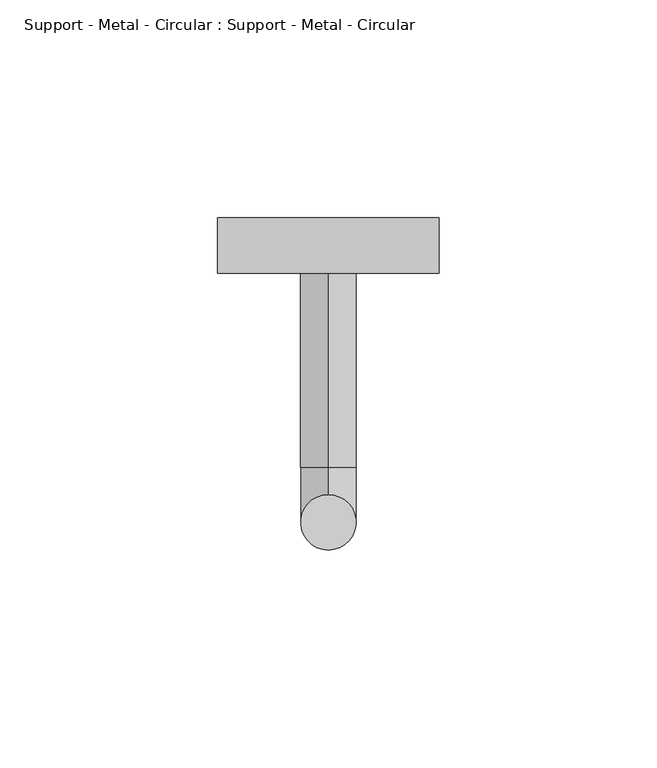
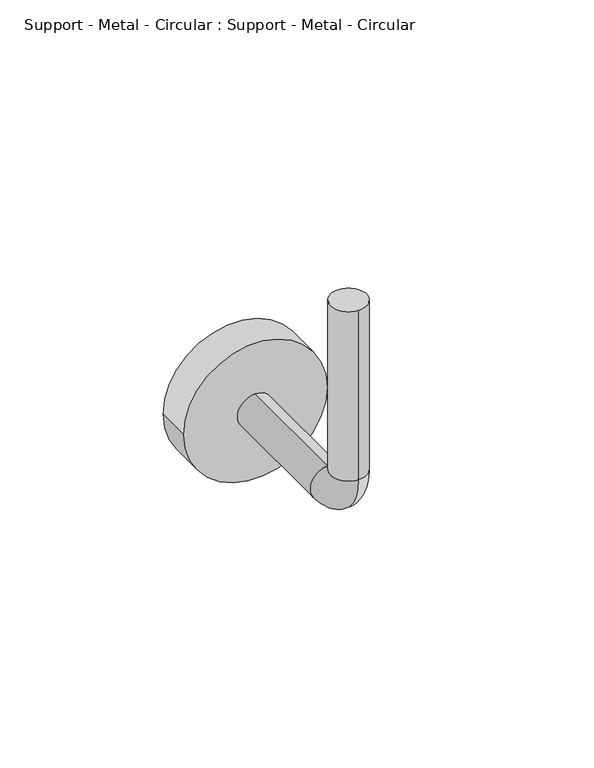
"""IFC4 building model written with IfcOpenShell, lengths in millimetres: proxy geometry, Support - Metal - Circular : Support - Metal - Circular."""

from ifc_helpers import new_model, si_unit, point, frame, frame_2d, origin, origin_with_axes, place, context, project, spatial, circle_curve, ellipse_curve, trimmed, segment, composite_curve, outline, extrude, source, transform, mapped, element, save
from ifc_brep_helpers import plane_surface, cylinder_surface, revolved_surface, advanced_brep


def support_metal_circular_support_metal_circular_b7c6dc0a(model_context):
    return source(origin(), model_context, "Body", "SolidModel", [
        advanced_brep(
        [(0.0, 57.15, -69.85), (0.0, 57.15, -82.55), (0.0, 12.7, -69.85), (0.0, 12.7, -82.55), (0.0, -6.35, -63.5), (0.0, 6.35, -63.5), (0.0, 6.35, 0.0), (0.0, -6.35, 0.0)],
        [
            (0, 1, circle_curve(frame((0.0, 57.15, -76.2), z_axis=(0.0, 1.0, 0.0), x_axis=(0.0, 0.0, -1.0)), 6.35)),
            (1, 0, circle_curve(frame((0.0, 57.15, -76.2), z_axis=(0.0, 1.0, 0.0), x_axis=(0.0, 0.0, -1.0)), 6.35)),
            (0, 2),
            (2, 3, circle_curve(frame((0.0, 12.7, -76.2), z_axis=(0.0, 1.0, 0.0), x_axis=(0.0, 0.0, -1.0)), 6.35)),
            (3, 1),
            (3, 2, circle_curve(frame((0.0, 12.7, -76.2), z_axis=(0.0, 1.0, 0.0), x_axis=(0.0, 0.0, -1.0)), 6.35)),
            (4, 3, circle_curve(frame((0.0, 12.7, -63.5), z_axis=(1.0, 0.0, 0.0), x_axis=(0.0, 0.0, -1.0)), 19.05)),
            (2, 5, circle_curve(frame((0.0, 12.7, -63.5), z_axis=(-1.0, 0.0, 0.0), x_axis=(0.0, 0.0, -1.0)), 6.35)),
            (5, 4, circle_curve(frame((0.0, 0.0, -63.5), z_axis=(0.0, 0.0, -1.0), x_axis=(0.0, -1.0, 0.0)), 6.35)),
            (4, 5, circle_curve(frame((0.0, 0.0, -63.5), z_axis=(0.0, 0.0, -1.0), x_axis=(0.0, -1.0, 0.0)), 6.35)),
            (6, 7, circle_curve(frame((0.0, 0.0, 0.0), z_axis=(0.0, 0.0, 1.0), x_axis=(0.0, -1.0, 0.0)), 6.35)),
            (7, 6, circle_curve(frame((0.0, 0.0, 0.0), z_axis=(0.0, 0.0, 1.0), x_axis=(0.0, -1.0, 0.0)), 6.35)),
            (5, 6),
            (7, 4),
        ],
        [
            plane_surface(frame((0.0, 57.15, -76.2), z_axis=(0.0, 1.0, 0.0), x_axis=(1.0, 0.0, 0.0))),
            cylinder_surface(frame((0.0, 57.15, -76.2), z_axis=(0.0, 1.0, 0.0), x_axis=(0.0, 0.0, -1.0)), 6.35),
            revolved_surface(trimmed(ellipse_curve(frame((0.0, 12.7, -76.2), z_axis=(0.0, 1.0, 0.0), x_axis=(0.0, 0.0, -1.0)), 6.35, 6.35), [point((0.0, 12.7, -69.85))], [point((0.0, 12.7, -82.55))], True, "CARTESIAN"), (0.0, 12.7, -63.5), (-1.0, 0.0, 0.0)),
            revolved_surface(trimmed(ellipse_curve(frame((0.0, 12.7, -76.2), z_axis=(0.0, 1.0, 0.0), x_axis=(0.0, 0.0, -1.0)), 6.35, 6.35), [point((0.0, 12.7, -82.55))], [point((0.0, 12.7, -69.85))], True, "CARTESIAN"), (0.0, 12.7, -63.5), (-1.0, 0.0, 0.0)),
            plane_surface(origin_with_axes()),
            cylinder_surface(frame((0.0, 0.0, -63.5), z_axis=(0.0, 0.0, -1.0), x_axis=(0.0, -1.0, 0.0)), 6.35),
        ],
        [
            (0, [[1, 2]]),
            (1, [[-1, 3, 4, 5]]),
            (1, [[-2, -5, 6, -3]]),
            (2, [[7, -4, 8, 9]]),
            (3, [[-8, -6, -7, 10]]),
            (4, [[11, 12]]),
            (5, [[-9, 13, -12, 14]]),
            (5, [[-10, -14, -11, -13]]),
        ],
    ),
        extrude(outline(composite_curve([segment(trimmed(circle_curve(frame_2d((-76.2, 0.0)), 25.4), [point((-76.2, -25.4))], [point((-76.2, 25.4))], False, "CARTESIAN"), True, "CONTINUOUS"), segment(trimmed(circle_curve(frame_2d((-76.2, 0.0)), 25.4), [point((-76.2, 25.4))], [point((-76.2, -25.4))], False, "CARTESIAN"), True, "CONTINUOUS")], self_intersect=False)), frame((0.0, 57.15, 0.0), z_axis=(0.0, 1.0, 0.0), x_axis=(0.0, 0.0, 1.0)), (0.0, 0.0, 1.0), 12.7),
    ])


if __name__ == "__main__":
    model = new_model("IFC4")
    model_context = context("Model", 3, world=origin())
    ifc_project = project(units=[si_unit("LENGTHUNIT", "METRE", prefix="MILLI")], contexts=[model_context])
    site = spatial("IfcSite", under=ifc_project)
    building = spatial("IfcBuilding", under=site)
    placement = place(None, origin())
    support_metal_circular_support_metal_circular_shape = support_metal_circular_support_metal_circular_b7c6dc0a(model_context)
    element("IfcBuildingElementProxy", 1, Name="Support - Metal - Circular : Support - Metal - Circular", ObjectType="Support - Metal - Circular : Support - Metal - Circular", at=placement, inside=building, context=model_context, shape_type="MappedRepresentation", body=[
        mapped(support_metal_circular_support_metal_circular_shape, transform((0.0, 0.0, 0.0), x_axis=(1.0, 0.0, 0.0), y_axis=(0.0, 1.0, 0.0), z_axis=(0.0, 0.0, 1.0))),
    ])
    save(model, "model.ifc")

# Revit data of these elements
# Type "Support - Metal - Circular : Support - Metal - Circular"
#   T1 = 0' - 0 1/2"
#   Radius 1 = 0' - 1"
#   Radius 2 = 0' - 0 1/4"
#   built-in parameter 1152166 = 0.25 (stored number, unit not read)
#   built-in parameter 1152165 [instance default] = 0.25 (stored number, unit not read)
#   Bend Radius = 0' - 0 1/2"
#   Support Material = KAWNEER TRIFAB VERSAGLAZE 451T - CLEAR ANODIZED ALUM. - BACK GLAZED
# Element 1 (IfcBuildingElementProxy, "Support - Metal - Circular : Support - Metal - Circular")
#   built-in parameter 1152165 = 0.229167 (stored number, unit not read)
#   Materials on its faces: "KAWNEER TRIFAB VERSAGLAZE 451T - CLEAR ANODIZED ALUM. - BACK GLAZED"
# Materials
#   "KAWNEER TRIFAB VERSAGLAZE 451T - CLEAR ANODIZED ALUM. - BACK GLAZED": class "Metal", colour RGB 244 244 244, transparency 0, Description = "Aluminum 6061", Cost = 0
